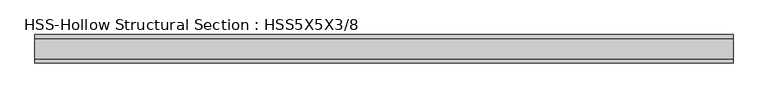
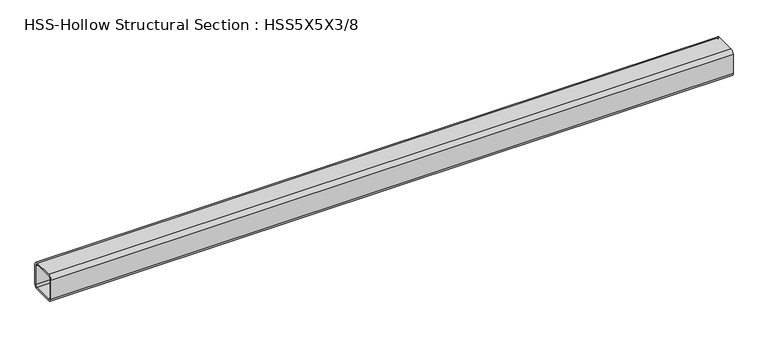
"""IFC4 building model written with IfcOpenShell, lengths in millimetres: member geometry, HSS-Hollow Structural Section : HSS5X5X3/8."""

from ifc_helpers import new_model, si_unit, point, frame, frame_2d, origin, place, context, project, spatial, polyline, circle_curve, trimmed, segment, composite_curve, outline, extrude, source, transform, mapped, element, save


def hss_hollow_structural_section_hss5x5x3_8_66eacc37(model_context):
    return source(origin(), model_context, "Body", "SweptSolid", [
        extrude(outline(composite_curve([segment(polyline([(63.5, 45.7708), (63.5, -45.7708)]), True, "CONTINUOUS"), segment(trimmed(circle_curve(frame_2d((45.7708, -45.7708)), 17.7292), [point((63.5, -45.7708))], [point((45.7708, -63.5))], False, "CARTESIAN"), True, "CONTINUOUS"), segment(polyline([(45.7708, -63.5), (-45.7708, -63.5)]), True, "CONTINUOUS"), segment(trimmed(circle_curve(frame_2d((-45.7708, -45.7708)), 17.7292), [point((-45.7708, -63.5))], [point((-63.5, -45.7708))], False, "CARTESIAN"), True, "CONTINUOUS"), segment(polyline([(-63.5, -45.7708), (-63.5, 45.7708)]), True, "CONTINUOUS"), segment(trimmed(circle_curve(frame_2d((-45.7708, 45.7708)), 17.7292), [point((-63.5, 45.7708))], [point((-45.7708, 63.5))], False, "CARTESIAN"), True, "CONTINUOUS"), segment(polyline([(-45.7708, 63.5), (45.7708, 63.5)]), True, "CONTINUOUS"), segment(trimmed(circle_curve(frame_2d((45.7708, 45.7708)), 17.7292), [point((45.7708, 63.5))], [point((63.5, 45.7708))], False, "CARTESIAN"), True, "CONTINUOUS")], self_intersect=False), holes=[composite_curve([segment(trimmed(circle_curve(frame_2d((-45.7708, 45.7708)), 8.8646), [point((-45.7708, 54.6354))], [point((-54.6354, 45.7708))], True, "CARTESIAN"), True, "CONTINUOUS"), segment(polyline([(-54.6354, 45.7708), (-54.6354, -45.7708)]), True, "CONTINUOUS"), segment(trimmed(circle_curve(frame_2d((-45.7708, -45.7708)), 8.8646), [point((-54.6354, -45.7708))], [point((-45.7708, -54.6354))], True, "CARTESIAN"), True, "CONTINUOUS"), segment(polyline([(-45.7708, -54.6354), (45.7708, -54.6354)]), True, "CONTINUOUS"), segment(trimmed(circle_curve(frame_2d((45.7708, -45.7708)), 8.8646), [point((45.7708, -54.6354))], [point((54.6354, -45.7708))], True, "CARTESIAN"), True, "CONTINUOUS"), segment(polyline([(54.6354, -45.7708), (54.6354, 45.7708)]), True, "CONTINUOUS"), segment(trimmed(circle_curve(frame_2d((45.7708, 45.7708)), 8.8646), [point((54.6354, 45.7708))], [point((45.7708, 54.6354))], True, "CARTESIAN"), True, "CONTINUOUS"), segment(polyline([(45.7708, 54.6354), (-45.7708, 54.6354)]), True, "CONTINUOUS")], self_intersect=False)]), frame((-1563.4187975, 0.0, 0.0), z_axis=(1.0, 0.0, 0.0), x_axis=(0.0, 1.0, 0.0)), (0.0, 0.0, 1.0), 3126.8375951),
    ])


if __name__ == "__main__":
    model = new_model("IFC4")
    model_context = context("Model", 3, world=origin())
    ifc_project = project(units=[si_unit("LENGTHUNIT", "METRE", prefix="MILLI")], contexts=[model_context])
    site = spatial("IfcSite", under=ifc_project)
    building = spatial("IfcBuilding", under=site)
    placement = place(None, origin())
    hss_hollow_structural_section_hss5x5x3_8_shape = hss_hollow_structural_section_hss5x5x3_8_66eacc37(model_context)
    element("IfcMember", 1, ObjectType="HSS-Hollow Structural Section : HSS5X5X3/8", at=placement, inside=building, context=model_context, shape_type="MappedRepresentation", body=[
        mapped(hss_hollow_structural_section_hss5x5x3_8_shape, transform((0.0, 0.0, 0.0), x_axis=(1.0, 0.0, 0.0), y_axis=(0.0, 1.0, 0.0), z_axis=(0.0, 0.0, 1.0))),
    ])
    save(model, "model.ifc")

# Revit data of these elements
# Type "HSS-Hollow Structural Section : HSS5X5X3/8"
#   Assembly Code = "B10"
#   Shape = "Square"
#   W = 22.3
#   Ht = 0' - 5"
#   Length [instance default] = 5' - 0"
#   b = 0' - 5"
#   kr = 0' - 0.698"
#   t = 0' - 0.349"
#   A = 0.0429167 SF
#   Structural Material [instance default] = Steel ASTM A500, Grade B, Rectangular and Square
# Element 1 (IfcMember, "HSS-Hollow Structural Section : HSS5X5X3/8")
#   Materials on its faces: "Steel ASTM A500, Grade B, Rectangular and Square"
# Materials
#   "Steel ASTM A500, Grade B, Rectangular and Square": class "Metal", colour RGB 199 199 199, transparency 0, Description = "Carbon steel", Cost = 0
